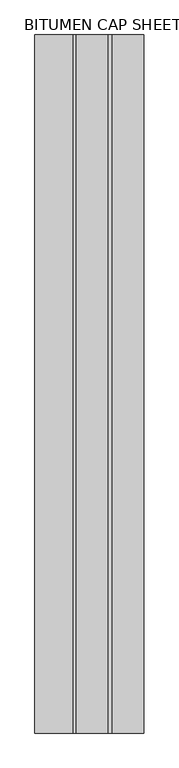
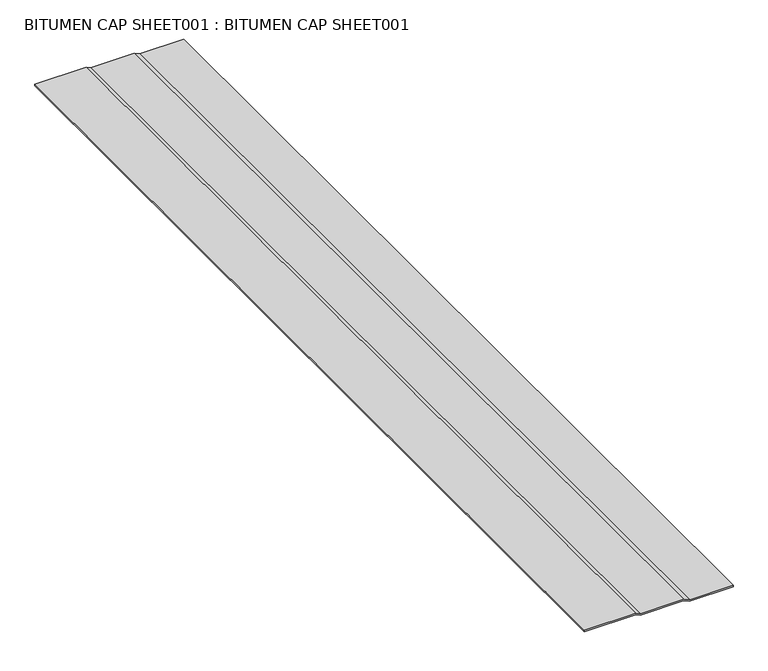
"""IFC4 building model written with IfcOpenShell, lengths in millimetres: proxy geometry, BITUMEN CAP SHEET001 : BITUMEN CAP SHEET001."""

import ifcopenshell
import ifcopenshell.guid

model = None  # the IFC model being written
_history = None  # IfcOwnerHistory: only IFC2X3 demands one
_inside = {}  # id of a spatial element -> (the spatial element, [elements in it])
_under = {}  # id of a project, library or spatial element -> (it, [spatial elements below it])
_declared = {}  # id of a project -> (the project, [libraries it declares])
_typed = {}  # id of a type object -> (the type object, [elements of that type])
_made_of = {}  # id of a material, layer set ... -> (it, [elements and type objects made of it])


def new_model(schema):
    """Start an empty IFC model of exactly this schema.

    Asked for "IFC4X3", IfcOpenShell would pick the latest addendum, in which some entities
    have other attributes; the version numbers below select the first issue.
    IFC2X3 requires an IfcOwnerHistory on every rooted entity: one is made here for all.
    """
    global model, _history
    if schema == "IFC4X3":
        model = ifcopenshell.file(schema_version=(4, 3, 0, 0))
    else:
        model = ifcopenshell.file(schema=schema)
    _inside.clear()
    _under.clear()
    _declared.clear()
    _typed.clear()
    _made_of.clear()
    _history = None
    if model.schema == "IFC2X3":
        org = make("IfcOrganization", Name="unknown")
        user = make(
            "IfcPersonAndOrganization",
            ThePerson=make("IfcPerson", FamilyName="unknown"),
            TheOrganization=org,
        )
        app = make(
            "IfcApplication",
            ApplicationDeveloper=org,
            Version="unknown",
            ApplicationFullName="unknown",
            ApplicationIdentifier="unknown",
        )
        _history = make(
            "IfcOwnerHistory",
            OwningUser=user,
            OwningApplication=app,
            ChangeAction="ADDED",
            CreationDate=0,
        )
    return model


def make(cls, **values):
    """One entity of the class cls with the attributes given. An attribute that is None is left unset."""
    return model.create_entity(
        cls, **{name: value for name, value in values.items() if value is not None}
    )


def rooted(cls, **values):
    """An entity with a GlobalId (a new one), such as an element, a storey or a relation."""
    return make(cls, GlobalId=ifcopenshell.guid.new(), OwnerHistory=_history, **values)


def si_unit(unit_type, name, prefix=None):
    """IfcSIUnit, for example si_unit("LENGTHUNIT", "METRE", prefix="MILLI")."""
    return make("IfcSIUnit", UnitType=unit_type, Prefix=prefix, Name=name)


def assignment(units):
    """IfcUnitAssignment: the units of a project."""
    return None if units is None else make("IfcUnitAssignment", Units=units)


def point(xyz):
    """IfcCartesianPoint."""
    return None if xyz is None else make("IfcCartesianPoint", Coordinates=xyz)


def direction(xyz):
    """IfcDirection."""
    return None if xyz is None else make("IfcDirection", DirectionRatios=xyz)


def frame(location, z_axis=None, x_axis=None):
    """IfcAxis2Placement3D, a coordinate frame: its origin and axes. An axis left out is left unset."""
    return make(
        "IfcAxis2Placement3D",
        Location=point(location),
        Axis=direction(z_axis),
        RefDirection=direction(x_axis),
    )


def origin():
    """The frame at (0, 0, 0) with its axes left unset."""
    return frame((0.0, 0.0, 0.0))


def place(relative_to, where):
    """IfcLocalPlacement: puts the frame where relative to a parent placement (None: the world)."""
    return make(
        "IfcLocalPlacement", PlacementRelTo=relative_to, RelativePlacement=where
    )


def context(
    kind, dimensions, precision=None, world=None, true_north=None, identifier=None
):
    """IfcGeometricRepresentationContext, for example the 3D "Model" context."""
    return make(
        "IfcGeometricRepresentationContext",
        ContextIdentifier=identifier,
        ContextType=kind,
        CoordinateSpaceDimension=dimensions,
        Precision=precision,
        WorldCoordinateSystem=world,
        TrueNorth=true_north,
    )


def project(units=None, contexts=None):
    """IfcProject with its units and contexts."""
    return rooted(
        "IfcProject",
        Name="project",
        RepresentationContexts=contexts,
        UnitsInContext=assignment(units),
    )


def spatial(cls, under=None, at=None, **own):
    """A site, building, storey or space (cls), placed at a placement, below another one or the project."""
    s = rooted(cls, ObjectPlacement=at, **own)
    if under is not None:
        _under.setdefault(under.id(), (under, []))[1].append(s)
    return s


def polyline(points):
    """IfcPolyline through the points."""
    return make("IfcPolyline", Points=[point(p) for p in points])


def outline(outer, holes=None, kind="AREA"):
    """IfcArbitraryClosedProfileDef: a profile drawn as a closed curve; with holes, ...WithVoids."""
    if holes is None:
        return make("IfcArbitraryClosedProfileDef", ProfileType=kind, OuterCurve=outer)
    return make(
        "IfcArbitraryProfileDefWithVoids",
        ProfileType=kind,
        OuterCurve=outer,
        InnerCurves=holes,
    )


def extrude(swept, where, along, depth):
    """IfcExtrudedAreaSolid: the profile swept, set in the frame where, extruded along a direction by depth."""
    return make(
        "IfcExtrudedAreaSolid",
        SweptArea=swept,
        Position=where,
        ExtrudedDirection=direction(along),
        Depth=depth,
    )


def shape(context_of_items, identifier, shape_type, items):
    """IfcShapeRepresentation: the items that make up one representation, for example the "Body"."""
    return make(
        "IfcShapeRepresentation",
        ContextOfItems=context_of_items,
        RepresentationIdentifier=identifier,
        RepresentationType=shape_type,
        Items=items,
    )


def source(mapping_origin, context_of_items, identifier, shape_type, items):
    """IfcRepresentationMap: a shape defined once, which mapped items show again and again."""
    return make(
        "IfcRepresentationMap",
        MappingOrigin=mapping_origin,
        MappedRepresentation=shape(context_of_items, identifier, shape_type, items),
    )


def transform(
    local_origin,
    x_axis=None,
    y_axis=None,
    z_axis=None,
    scale=None,
    scale2=None,
    scale3=None,
    uniform=True,
):
    """IfcCartesianTransformationOperator3D, or its non-uniform kind. x_axis, y_axis, z_axis: its Axis1, 2, 3."""
    if uniform:
        return make(
            "IfcCartesianTransformationOperator3D",
            Axis1=direction(x_axis),
            Axis2=direction(y_axis),
            LocalOrigin=point(local_origin),
            Scale=scale,
            Axis3=direction(z_axis),
        )
    return make(
        "IfcCartesianTransformationOperator3DnonUniform",
        Axis1=direction(x_axis),
        Axis2=direction(y_axis),
        LocalOrigin=point(local_origin),
        Scale=scale,
        Axis3=direction(z_axis),
        Scale2=scale2,
        Scale3=scale3,
    )


def mapped(mapping_source, mapping_target):
    """IfcMappedItem: shows the shape of a source again, moved by a transform."""
    return make(
        "IfcMappedItem", MappingSource=mapping_source, MappingTarget=mapping_target
    )


def made_of(thing, what):
    """Note that an element or type object is made of a material, layer set ...; save() writes the relation."""
    if what is not None:
        _made_of.setdefault(what.id(), (what, []))[1].append(thing)
    return thing


def element(
    cls,
    number,
    at=None,
    inside=None,
    cuts=None,
    type_object=None,
    material=None,
    context=None,
    identifier="Body",
    shape_type=None,
    held_by="IfcProductDefinitionShape",
    body=None,
    shapes=None,
    **own,
):
    """One element of the class cls, such as IfcWall. Its Tag is "e" and its number.

    at: its placement. inside: the storey or other place that contains it. cuts: it is an
    opening in that element (IfcRelVoidsElement). A single representation is given by context,
    identifier, shape_type and body (its items); several are given by shapes. held_by: the class
    of the entity that holds the representations. save() writes the other relations.
    """
    e = rooted(cls, Tag="e%d" % number, ObjectPlacement=at, **own)
    if body is not None:
        shapes = [shape(context, identifier, shape_type, body)]
    if shapes is not None:
        e.Representation = make(held_by, Representations=shapes)
    if inside is not None:
        _inside.setdefault(inside.id(), (inside, []))[1].append(e)
    if cuts is not None:
        rooted(
            "IfcRelVoidsElement", RelatingBuildingElement=cuts, RelatedOpeningElement=e
        )
    if type_object is not None:
        _typed.setdefault(type_object.id(), (type_object, []))[1].append(e)
    return made_of(e, material)


def aggregate(whole, parts):
    """IfcRelAggregates: a whole, such as a stair, and the parts it consists of."""
    return rooted("IfcRelAggregates", RelatingObject=whole, RelatedObjects=parts)


def save(model, path):
    """Write the relations noted so far, then the file.

    IfcRelAggregates (storeys below a building ...), IfcRelContainedInSpatialStructure (elements
    in a storey), IfcRelDefinesByType, IfcRelAssociatesMaterial and IfcRelDeclares: one each for
    every whole, place, type object, material and project.
    """
    for whole, parts in _under.values():
        aggregate(whole, parts)
    for where, things in _inside.values():
        rooted(
            "IfcRelContainedInSpatialStructure",
            RelatedElements=things,
            RelatingStructure=where,
        )
    for kind, things in _typed.values():
        rooted("IfcRelDefinesByType", RelatedObjects=things, RelatingType=kind)
    for what, things in _made_of.values():
        rooted("IfcRelAssociatesMaterial", RelatedObjects=things, RelatingMaterial=what)
    for by, libraries in _declared.values():
        rooted("IfcRelDeclares", RelatingContext=by, RelatedDefinitions=libraries)
    model.write(path)


def bitumen_cap_sheet001_bitumen_cap_sheet001_3f8c56e2(model_context):
    return source(origin(), model_context, "Body", "SweptSolid", [
        extrude(outline(polyline([(40259.2002678, -4699.8063764), (40262.3752678, -4699.8063764), (40262.3752678, -4791.325638), (40267.6612773, -4803.7904566), (40267.6612773, -4894.4742123), (40271.9940719, -4904.1911138), (40271.9940719, -5012.0776104), (40268.8188423, -5012.0776104), (40268.8188423, -4904.8663993), (40264.4862773, -4895.1500128), (40264.4862773, -4804.4358566), (40259.2002678, -4791.971038), (40259.2002678, -4699.8063764)])), frame((0.0, -1052.8906574, 0.0), z_axis=(0.0, 1.0, 0.0), x_axis=(0.0, 0.0, 1.0)), (0.0, 0.0, 1.0), 2000.25),
    ])


if __name__ == "__main__":
    model = new_model("IFC4")
    model_context = context("Model", 3, world=origin())
    ifc_project = project(units=[si_unit("LENGTHUNIT", "METRE", prefix="MILLI")], contexts=[model_context])
    site = spatial("IfcSite", under=ifc_project)
    building = spatial("IfcBuilding", under=site)
    placement = place(None, origin())
    bitumen_cap_sheet001_bitumen_cap_sheet001_shape = bitumen_cap_sheet001_bitumen_cap_sheet001_3f8c56e2(model_context)
    element("IfcBuildingElementProxy", 1, Name="BITUMEN CAP SHEET001 : BITUMEN CAP SHEET001", ObjectType="BITUMEN CAP SHEET001 : BITUMEN CAP SHEET001", at=placement, inside=building, context=model_context, shape_type="MappedRepresentation", body=[
        mapped(bitumen_cap_sheet001_bitumen_cap_sheet001_shape, transform((0.0, 0.0, 0.0), x_axis=(1.0, 0.0, 0.0), y_axis=(0.0, 1.0, 0.0), z_axis=(0.0, 0.0, 1.0))),
    ])
    save(model, "model.ifc")

# Revit data of these elements
# Type "BITUMEN CAP SHEET001 : BITUMEN CAP SHEET001"
#   NameOverride = "BITUMEN CAP SHEET001"
# Element 1 (IfcBuildingElementProxy, "BITUMEN CAP SHEET001 : BITUMEN CAP SHEET001")
#   Materials on its faces: "MODIFIED BITUMEN GRANULE SURFACED CAP SHEET"
# Materials
#   "MODIFIED BITUMEN GRANULE SURFACED CAP SHEET": class "Unassigned", colour RGB 85 85 127, transparency 0
